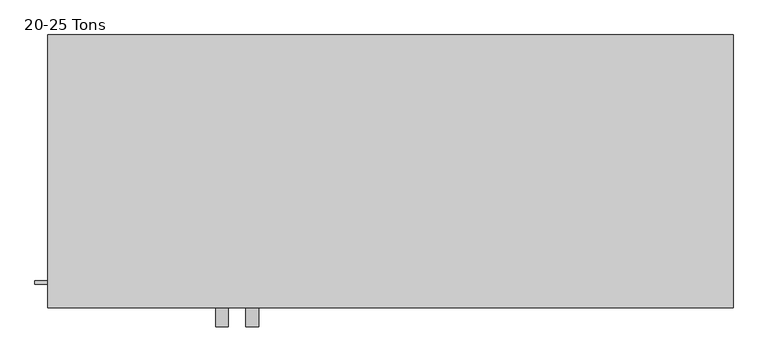
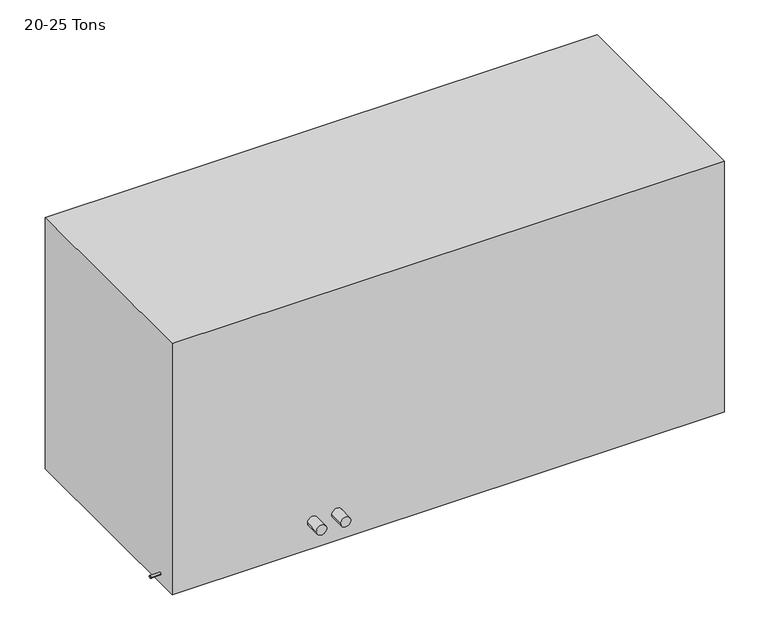
"""IFC4 building model written with IfcOpenShell, lengths in millimetres: proxy geometry, 20-55 Tons Air Cooled Scroll Chiller : 20-25 Tons."""

from ifc_helpers import new_model, si_unit, frame, origin, place, context, project, spatial, circle_curve, source, transform, mapped, element, save
from ifc_brep_helpers import plane_surface, cylinder_surface, advanced_brep


def proxy_20_25_tons_50dc316f(model_context):
    return source(origin(), model_context, "Body", "AdvancedBrep", [
        advanced_brep(
        [(2743.2, 0.0, 1320.8), (0.0, 0.0, 1320.8), (0.0, -1092.2, 1320.8), (2743.2, -1092.2, 1320.8), (2743.2, 0.0, 0.0), (2743.2, -1092.2, 0.0), (0.0, -1092.2, 0.0), (0.0, 0.0, 0.0), (0.0, -996.95, 50.8), (0.0, -984.25, 50.8), (723.9, -1092.2, 142.875), (673.1, -1092.2, 142.875), (844.55, -1092.2, 142.875), (793.75, -1092.2, 142.875), (-50.8, -996.95, 50.8), (-50.8, -984.25, 50.8), (673.1, -1168.4, 142.875), (723.9, -1168.4, 142.875), (793.75, -1168.4, 142.875), (844.55, -1168.4, 142.875)],
        [
            (0, 1),
            (1, 2),
            (2, 3),
            (3, 0),
            (4, 5),
            (5, 6),
            (6, 7),
            (7, 4),
            (0, 4),
            (7, 1),
            (6, 2),
            (8, 9, circle_curve(frame((0.0, -990.6, 50.8), z_axis=(1.0, 0.0, 0.0), x_axis=(0.0, 1.0, 0.0)), 6.35)),
            (9, 8, circle_curve(frame((0.0, -990.6, 50.8), z_axis=(1.0, 0.0, 0.0), x_axis=(0.0, 1.0, 0.0)), 6.35)),
            (5, 3),
            (10, 11, circle_curve(frame((698.5, -1092.2, 142.875), z_axis=(0.0, 1.0, 0.0), x_axis=(1.0, 0.0, 0.0)), 25.4)),
            (11, 10, circle_curve(frame((698.5, -1092.2, 142.875), z_axis=(0.0, 1.0, 0.0), x_axis=(1.0, 0.0, 0.0)), 25.4)),
            (12, 13, circle_curve(frame((819.15, -1092.2, 142.875), z_axis=(0.0, 1.0, 0.0), x_axis=(1.0, 0.0, 0.0)), 25.4)),
            (13, 12, circle_curve(frame((819.15, -1092.2, 142.875), z_axis=(0.0, 1.0, 0.0), x_axis=(1.0, 0.0, 0.0)), 25.4)),
            (14, 15, circle_curve(frame((-50.8, -990.6, 50.8), z_axis=(-1.0, 0.0, 0.0), x_axis=(0.0, 1.0, 0.0)), 6.35)),
            (15, 14, circle_curve(frame((-50.8, -990.6, 50.8), z_axis=(-1.0, 0.0, 0.0), x_axis=(0.0, 1.0, 0.0)), 6.35)),
            (15, 9),
            (8, 14),
            (16, 17, circle_curve(frame((698.5, -1168.4, 142.875), z_axis=(0.0, -1.0, 0.0), x_axis=(1.0, 0.0, 0.0)), 25.4)),
            (17, 16, circle_curve(frame((698.5, -1168.4, 142.875), z_axis=(0.0, -1.0, 0.0), x_axis=(1.0, 0.0, 0.0)), 25.4)),
            (16, 11),
            (10, 17),
            (18, 19, circle_curve(frame((819.15, -1168.4, 142.875), z_axis=(0.0, -1.0, 0.0), x_axis=(1.0, 0.0, 0.0)), 25.4)),
            (19, 18, circle_curve(frame((819.15, -1168.4, 142.875), z_axis=(0.0, -1.0, 0.0), x_axis=(1.0, 0.0, 0.0)), 25.4)),
            (18, 13),
            (12, 19),
        ],
        [
            plane_surface(frame((0.0, 0.0, 1320.8), z_axis=(0.0, 0.0, 1.0), x_axis=(-1.0, 0.0, 0.0))),
            plane_surface(frame((0.0, 0.0, 0.0), z_axis=(0.0, 0.0, -1.0), x_axis=(1.0, 0.0, 0.0))),
            plane_surface(frame((2743.2, 0.0, 1320.8), z_axis=(0.0, 1.0, 0.0), x_axis=(0.0, 0.0, -1.0))),
            plane_surface(frame((0.0, 0.0, 1320.8), z_axis=(-1.0, 0.0, 0.0), x_axis=(0.0, 0.0, -1.0))),
            plane_surface(frame((0.0, -1092.2, 1320.8), z_axis=(0.0, -1.0, 0.0), x_axis=(0.0, 0.0, -1.0))),
            plane_surface(frame((2743.2, -1092.2, 1320.8), z_axis=(1.0, 0.0, 0.0), x_axis=(0.0, 0.0, -1.0))),
            plane_surface(frame((-50.8, -984.25, 50.8), z_axis=(-1.0, 0.0, 0.0), x_axis=(0.0, 0.0, -1.0))),
            cylinder_surface(frame((-50.8, -990.6, 50.8), z_axis=(1.0, 0.0, 0.0), x_axis=(0.0, 1.0, 0.0)), 6.35),
            plane_surface(frame((723.9, -1168.4, 142.875), z_axis=(0.0, -1.0, 0.0), x_axis=(0.0, 0.0, 1.0))),
            cylinder_surface(frame((698.5, -1092.2, 142.875), z_axis=(0.0, -1.0, 0.0), x_axis=(1.0, 0.0, 0.0)), 25.4),
            plane_surface(frame((844.55, -1168.4, 142.875), z_axis=(0.0, -1.0, 0.0), x_axis=(0.0, 0.0, 1.0))),
            cylinder_surface(frame((819.15, -1092.2, 142.875), z_axis=(0.0, -1.0, 0.0), x_axis=(1.0, 0.0, 0.0)), 25.4),
        ],
        [
            (0, [[1, 2, 3, 4]]),
            (1, [[5, 6, 7, 8]]),
            (2, [[-1, 9, -8, 10]]),
            (3, [[-2, -10, -7, 11], [12, 13]]),
            (4, [[-3, -11, -6, 14], [15, 16], [17, 18]]),
            (5, [[-4, -14, -5, -9]]),
            (6, [[19, 20]]),
            (7, [[-20, 21, -12, 22]]),
            (7, [[-19, -22, -13, -21]]),
            (8, [[23, 24]]),
            (9, [[-23, 25, -15, 26]]),
            (9, [[-24, -26, -16, -25]]),
            (10, [[27, 28]]),
            (11, [[-27, 29, -17, 30]]),
            (11, [[-28, -30, -18, -29]]),
        ],
    ),
    ])


if __name__ == "__main__":
    model = new_model("IFC4")
    model_context = context("Model", 3, world=origin())
    ifc_project = project(units=[si_unit("LENGTHUNIT", "METRE", prefix="MILLI")], contexts=[model_context])
    site = spatial("IfcSite", under=ifc_project)
    building = spatial("IfcBuilding", under=site)
    placement = place(None, origin())
    proxy_20_25_tons_shape = proxy_20_25_tons_50dc316f(model_context)
    element("IfcBuildingElementProxy", 1, Name="20-55 Tons Air Cooled Scroll Chiller : 20-25 Tons", ObjectType="20-55 Tons Air Cooled Scroll Chiller : 20-25 Tons", at=placement, inside=building, context=model_context, shape_type="MappedRepresentation", body=[
        mapped(proxy_20_25_tons_shape, transform((0.0, 0.0, 0.0), x_axis=(1.0, 0.0, 0.0), y_axis=(0.0, 1.0, 0.0), z_axis=(0.0, 0.0, 1.0))),
    ])
    save(model, "model.ifc")

# Revit data of these elements
# Type "20-55 Tons Air Cooled Scroll Chiller : 20-25 Tons"
#   Voltage = 380 V
#   Pressure Drop [instance default] = 4.684 psi
#   Cooling Capacity [instance default] = 285584.4 Btu/h
#   Chiller Width = 3' - 7"
#   Chilled Water Supply Radius = 1"
#   Chilled Water Supply Diameter = 2"
#   Chilled Water Return Radius = 1"
#   Chilled Water Return Diameter = 2"
#   Chilled Water Flow [instance default] = 57 GPM
#   Apparent Load [instance default] = 29600 VA
#   visible 2 = no
#   visible 1 = no
#   visible 3 = yes
#   Number of Poles = 3
#   Chiller Material = none
# Element 1 (IfcBuildingElementProxy, "20-55 Tons Air Cooled Scroll Chiller : 20-25 Tons")
#   Chilled Water Flow = 0 GPM
